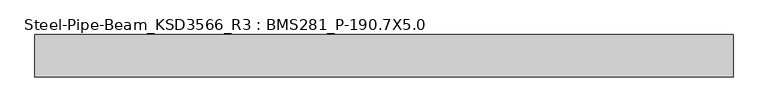
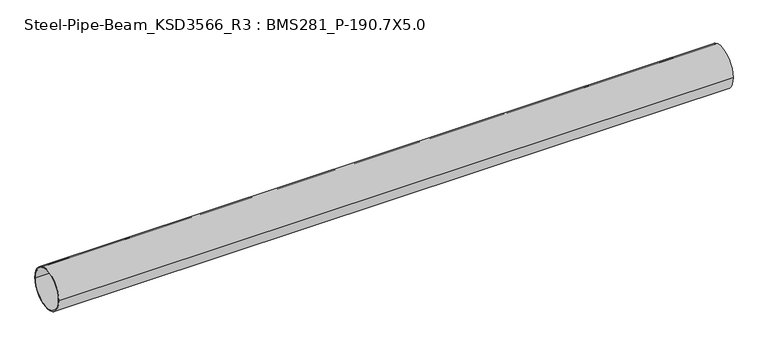
"""IFC4 building model written with IfcOpenShell, lengths in millimetres: member geometry, Steel-Pipe-Beam_KSD3566_R3 : BMS281_P-190.7X5.0."""

from ifc_helpers import new_model, si_unit, point, frame, origin, origin_2d, place, context, project, spatial, circle_curve, trimmed, segment, composite_curve, outline, extrude, source, transform, mapped, element, save


def steel_pipe_beam_ksd3566_r3_bms281_p_190_7x5_0_e6546c77(model_context):
    return source(origin(), model_context, "Body", "SweptSolid", [
        extrude(outline(composite_curve([segment(trimmed(circle_curve(origin_2d(), 95.35), [point((-95.35, 0.0))], [point((95.35, 0.0))], False, "CARTESIAN"), True, "CONTINUOUS"), segment(trimmed(circle_curve(origin_2d(), 95.35), [point((95.35, 0.0))], [point((-95.35, 0.0))], False, "CARTESIAN"), True, "CONTINUOUS")], self_intersect=False), holes=[composite_curve([segment(trimmed(circle_curve(origin_2d(), 90.35), [point((90.35, 0.0))], [point((-90.35, 0.0))], True, "CARTESIAN"), True, "CONTINUOUS"), segment(trimmed(circle_curve(origin_2d(), 90.35), [point((-90.35, 0.0))], [point((90.35, 0.0))], True, "CARTESIAN"), True, "CONTINUOUS")], self_intersect=False)]), frame((-1516.0407252, 0.0, 0.0), z_axis=(1.0, 0.0, 0.0), x_axis=(0.0, 1.0, 0.0)), (0.0, 0.0, 1.0), 3133.1971631),
    ])


if __name__ == "__main__":
    model = new_model("IFC4")
    model_context = context("Model", 3, world=origin())
    ifc_project = project(units=[si_unit("LENGTHUNIT", "METRE", prefix="MILLI")], contexts=[model_context])
    site = spatial("IfcSite", under=ifc_project)
    building = spatial("IfcBuilding", under=site)
    placement = place(None, origin())
    steel_pipe_beam_ksd3566_r3_bms281_p_190_7x5_0_shape = steel_pipe_beam_ksd3566_r3_bms281_p_190_7x5_0_e6546c77(model_context)
    element("IfcMember", 1, ObjectType="Steel-Pipe-Beam_KSD3566_R3 : BMS281_P-190.7X5.0", at=placement, inside=building, context=model_context, shape_type="MappedRepresentation", body=[
        mapped(steel_pipe_beam_ksd3566_r3_bms281_p_190_7x5_0_shape, transform((0.0, 0.0, 0.0), x_axis=(1.0, 0.0, 0.0), y_axis=(0.0, 1.0, 0.0), z_axis=(0.0, 0.0, 1.0))),
    ])
    save(model, "model.ifc")

# Revit data of these elements
# Type "Steel-Pipe-Beam_KSD3566_R3 : BMS281_P-190.7X5.0"
#   Keynote = "P-190.7X5.0"
#   SteelWeight = "Light"
#   t = 0.0050 m
#   Surface Area = 0.599102 m²/m
#   Section Area = 29.1697 cm²
#   Mass per Unit Length = 22.8982 kg/m
#   Length [instance default] = 1.5000 m
#   D = 0.1907 m
#   hec_material4 [instance default] = none
#   hec_material3 [instance default] = none
#   hec_material2 [instance default] = none
#   hec_material1 [instance default] = none
#   Structural Material [instance default] = Steel, 45-345
#   Assembly Code = ""
# Element 1 (IfcMember, "Steel-Pipe-Beam_KSD3566_R3 : BMS281_P-190.7X5.0")
#   Structural Material = none
# Materials
#   "Steel, 45-345": class "Metal", colour RGB 189 187 185, transparency 0, Description = "Steel 345 MPa", Cost = 0
